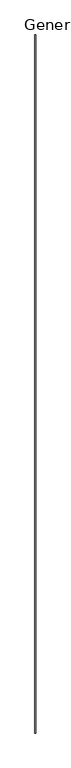
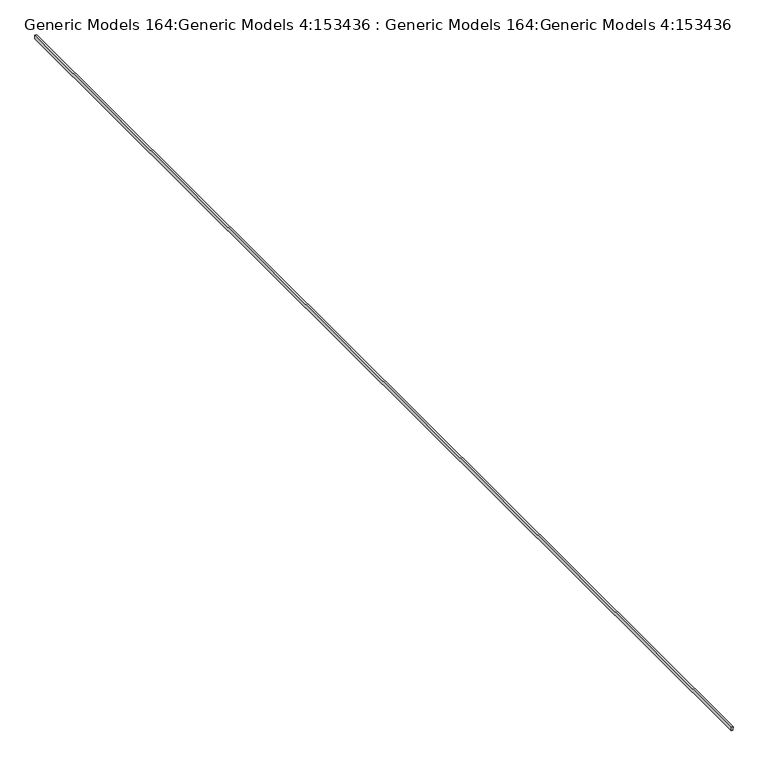
"""IFC4 building model written with IfcOpenShell, lengths in millimetres: proxy geometry, Generic Models 164:Generic Models 4:153436 : Generic Models 164:Generic Models 4:153436."""

from ifc_helpers import new_model, si_unit, frame, origin, place, context, project, spatial, polyline, outline, extrude, source, transform, mapped, element, save


def generic_models_164_generic_models_4_153436_generic_models_be2c52d2(model_context):
    return source(origin(), model_context, "Body", "SweptSolid", [
        extrude(outline(polyline([(-342.0475126, -10277.3328813), (-342.0475126, -10294.1571126), (-378.67399, -10294.1571126), (-378.67399, -10278.9203813), (-351.5725126, -10278.9203813), (-351.5725126, -10277.3328813), (-342.0475126, -10277.3328813)])), frame((0.0, -5303.1974793, 0.0), z_axis=(0.0, 1.0, 0.0), x_axis=(0.0, 0.0, 1.0)), (0.0, 0.0, 1.0), 12547.6),
    ])


if __name__ == "__main__":
    model = new_model("IFC4")
    model_context = context("Model", 3, world=origin())
    ifc_project = project(units=[si_unit("LENGTHUNIT", "METRE", prefix="MILLI")], contexts=[model_context])
    site = spatial("IfcSite", under=ifc_project)
    building = spatial("IfcBuilding", under=site)
    placement = place(None, origin())
    generic_models_164_generic_models_4_153436_generic_models_shape = generic_models_164_generic_models_4_153436_generic_models_be2c52d2(model_context)
    element("IfcBuildingElementProxy", 1, Name="Generic Models 164:Generic Models 4:153436 : Generic Models 164:Generic Models 4:153436", ObjectType="Generic Models 164:Generic Models 4:153436 : Generic Models 164:Generic Models 4:153436", at=placement, inside=building, context=model_context, shape_type="MappedRepresentation", body=[
        mapped(generic_models_164_generic_models_4_153436_generic_models_shape, transform((0.0, 0.0, 0.0), x_axis=(1.0, 0.0, 0.0), y_axis=(0.0, 1.0, 0.0), z_axis=(0.0, 0.0, 1.0))),
    ])
    save(model, "model.ifc")

# Revit data of these elements
# Type "Generic Models 164:Generic Models 4:153436 : Generic Models 164:Generic Models 4:153436"
#   NameOverride = "Generic Models 164:Generic Models 4:153436"
#   ObjectTypeOverride = "Generic Models 164:Generic Models 4"
#   Reference = "Generic Models 4"
#   Category = "Generic Models"
#   Tag = "153436"
# Element 1 (IfcBuildingElementProxy, "Generic Models 164:Generic Models 4:153436 : Generic Models 164:Generic Models 4:153436")
#   Materials on its faces: "_MORTAR SETTING BED 12838"
# Materials
#   "_MORTAR SETTING BED 12838": class "Unassigned", colour RGB 191 191 191, transparency 0
